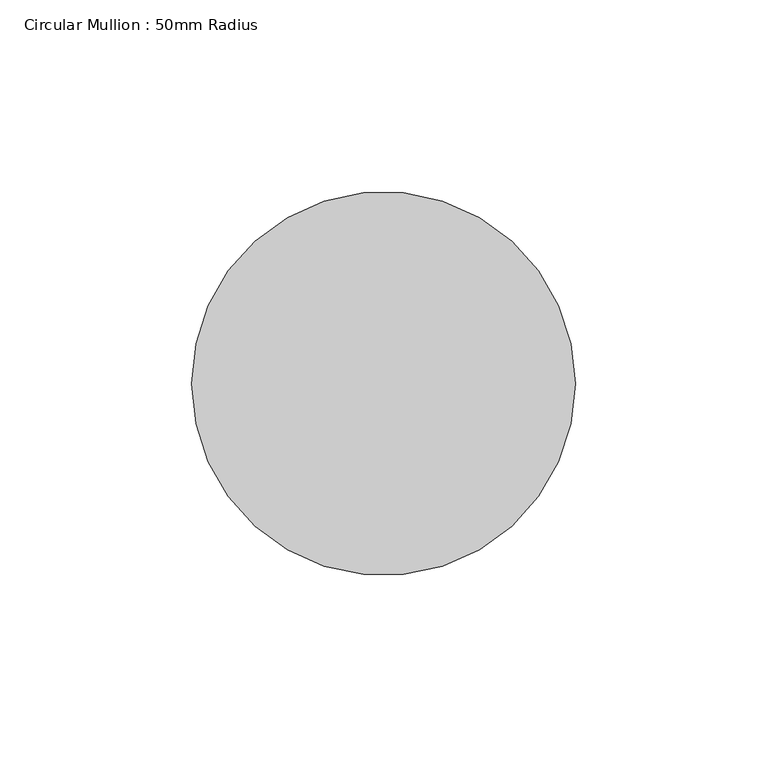
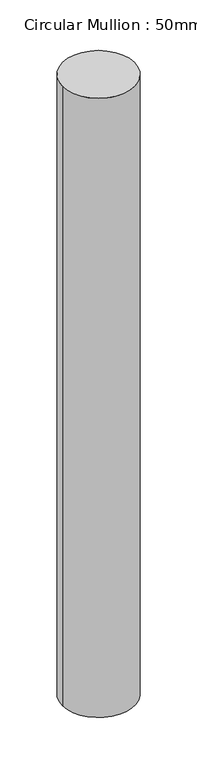
"""IFC4 building model written with IfcOpenShell, lengths in millimetres: member geometry, Circular Mullion : 50mm Radius."""

from ifc_helpers import new_model, si_unit, point, frame, origin, origin_2d, place, context, project, spatial, circle_curve, trimmed, segment, composite_curve, outline, extrude, source, transform, mapped, element, save


def circular_mullion_50mm_radius_d0940f0d(model_context):
    return source(origin(), model_context, "Body", "SweptSolid", [
        extrude(outline(composite_curve([segment(trimmed(circle_curve(origin_2d(), 50.0), [point((50.0, 0.0))], [point((-50.0, 0.0))], False, "CARTESIAN"), True, "CONTINUOUS"), segment(trimmed(circle_curve(origin_2d(), 50.0), [point((-50.0, 0.0))], [point((50.0, 0.0))], False, "CARTESIAN"), True, "CONTINUOUS")], self_intersect=False)), frame((0.0, 0.0, -905.5444602), z_axis=(0.0, 0.0, 1.0), x_axis=(1.0, 0.0, 0.0)), (0.0, 0.0, 1.0), 905.5444602),
    ])


if __name__ == "__main__":
    model = new_model("IFC4")
    model_context = context("Model", 3, world=origin())
    ifc_project = project(units=[si_unit("LENGTHUNIT", "METRE", prefix="MILLI")], contexts=[model_context])
    site = spatial("IfcSite", under=ifc_project)
    building = spatial("IfcBuilding", under=site)
    placement = place(None, origin())
    circular_mullion_50mm_radius_shape = circular_mullion_50mm_radius_d0940f0d(model_context)
    element("IfcMember", 1, ObjectType="Circular Mullion : 50mm Radius", at=placement, inside=building, context=model_context, shape_type="MappedRepresentation", body=[
        mapped(circular_mullion_50mm_radius_shape, transform((0.0, 0.0, 0.0), x_axis=(1.0, 0.0, 0.0), y_axis=(0.0, 1.0, 0.0), z_axis=(0.0, 0.0, 1.0))),
    ])
    save(model, "model.ifc")

# Revit data of these elements
# Type "Circular Mullion : 50mm Radius"
#   built-in parameter 1007350 = 0.164042 (stored number, unit not read)
# Element 1 (IfcMember, "Circular Mullion : 50mm Radius")
#   Materials on its faces: "Aluminium"
# Materials
#   "Aluminium": class "Metal", colour RGB 247 247 247, transparency 0, Description = "Aluminium 6061", Cost = 0
